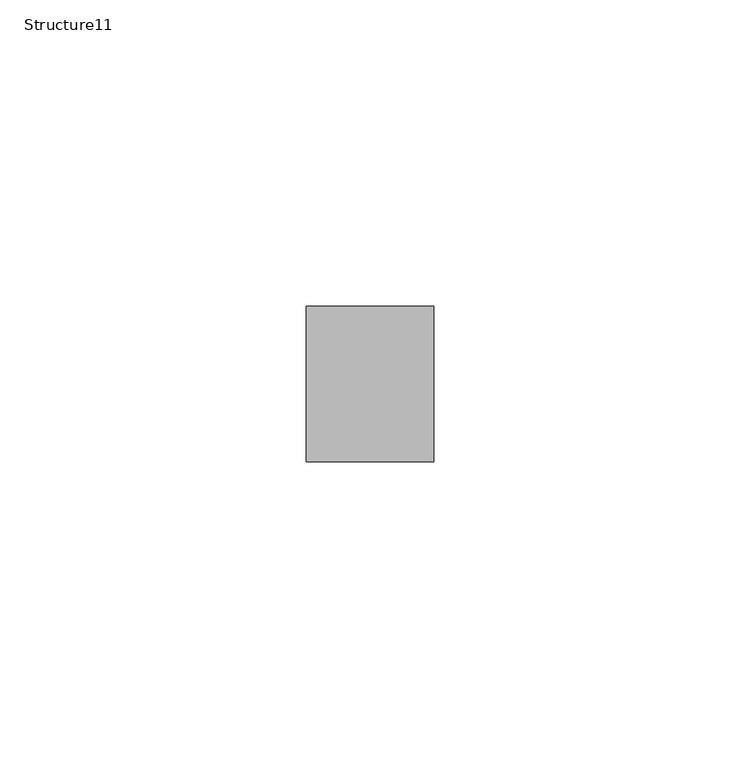
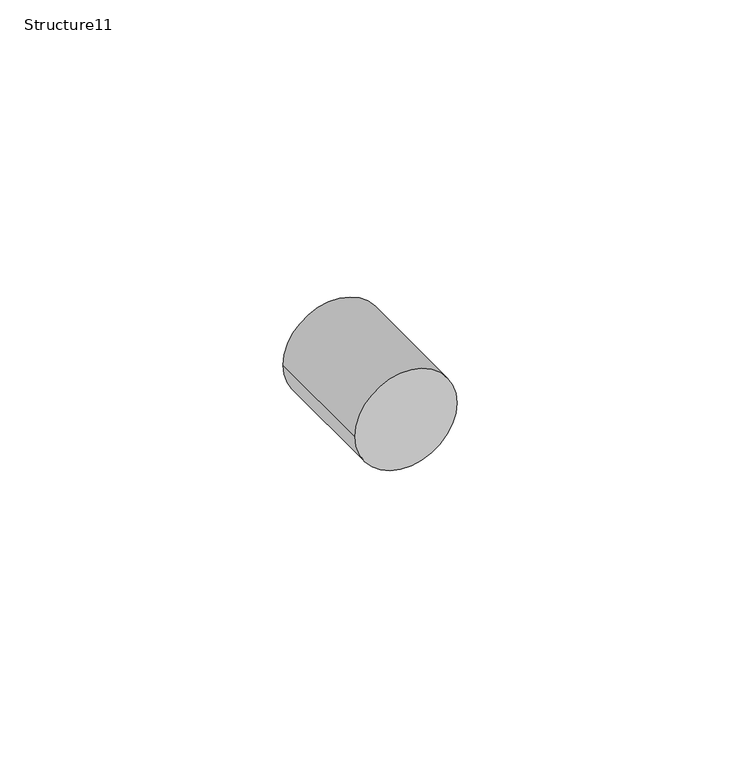
"""IFC4 building model written with IfcOpenShell, lengths in millimetres: proxy geometry, Structure11 : Structure668217132."""

from ifc_helpers import new_model, si_unit, point, frame, frame_2d, origin, place, context, project, spatial, circle_curve, trimmed, segment, composite_curve, outline, extrude, source, transform, mapped, element, save


def structure11_94f95103(model_context):
    return source(origin(), model_context, "Body", "SweptSolid", [
        extrude(outline(composite_curve([segment(trimmed(circle_curve(frame_2d((39371.6422813, 7343.0332877)), 10.4009751), [point((39371.6422813, 7332.6323126))], [point((39371.6422813, 7353.4342628))], False, "CARTESIAN"), True, "CONTINUOUS"), segment(trimmed(circle_curve(frame_2d((39371.6422813, 7343.0332877)), 10.4009751), [point((39371.6422813, 7353.4342628))], [point((39371.6422813, 7332.6323126))], False, "CARTESIAN"), True, "CONTINUOUS")], self_intersect=False)), frame((0.0, 1934.5461961, 0.0), z_axis=(0.0, 1.0, 0.0), x_axis=(0.0, 0.0, 1.0)), (0.0, 0.0, 1.0), 25.4),
    ])


if __name__ == "__main__":
    model = new_model("IFC4")
    model_context = context("Model", 3, world=origin())
    ifc_project = project(units=[si_unit("LENGTHUNIT", "METRE", prefix="MILLI")], contexts=[model_context])
    site = spatial("IfcSite", under=ifc_project)
    building = spatial("IfcBuilding", under=site)
    placement = place(None, origin())
    structure11_shape = structure11_94f95103(model_context)
    element("IfcBuildingElementProxy", 1, Name="Structure11 : Structure668217132", ObjectType="Structure11 : Structure668217132", at=placement, inside=building, context=model_context, shape_type="MappedRepresentation", body=[
        mapped(structure11_shape, transform((0.0, 0.0, 0.0), x_axis=(1.0, 0.0, 0.0), y_axis=(0.0, 1.0, 0.0), z_axis=(0.0, 0.0, 1.0))),
    ])
    save(model, "model.ifc")

# Revit data of these elements
# Type "Structure11 : Structure668217132"
#   NameOverride = "Structure668217132"
# Element 1 (IfcBuildingElementProxy, "Structure11 : Structure668217132")
#   Materials on its faces: "1.5\" DIA. STAINLESS STEEL RAILING"
# Materials
#   "1.5\" DIA. STAINLESS STEEL RAILING": class "Unassigned", colour RGB 128 128 128, transparency 0, Cost = 0
